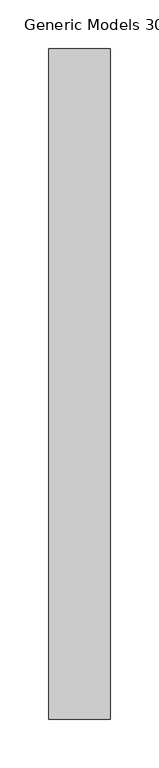
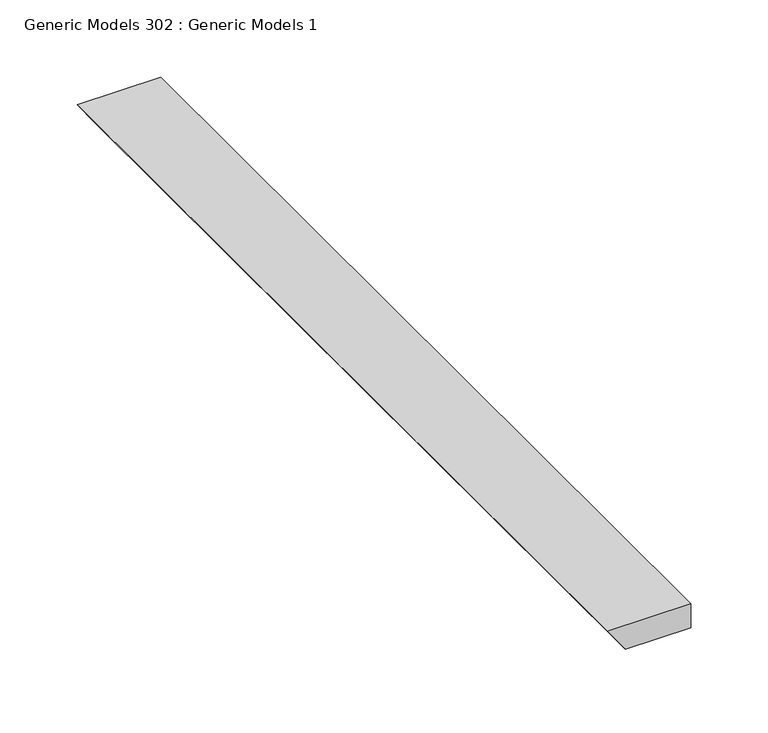
"""IFC4 building model written with IfcOpenShell, lengths in millimetres: proxy geometry, Generic Models 302 : Generic Models 1."""

from ifc_helpers import new_model, si_unit, frame, origin, place, context, project, spatial, polyline, outline, extrude, source, transform, mapped, element, save


def generic_models_302_generic_models_1_691b8c8b(model_context):
    return source(origin(), model_context, "Body", "SweptSolid", [
        extrude(outline(polyline([(124910.8145086, 4830.4400913), (124910.8145086, 4767.9223052), (124891.7645086, 4781.3763704), (124891.7645086, 4830.4400913), (124910.8145086, 4830.4400913)])), frame((0.0, 399.7309662, 0.0), z_axis=(0.0, 1.0, 0.0), x_axis=(0.0, 0.0, 1.0)), (0.0, 0.0, 1.0), 685.546),
    ])


if __name__ == "__main__":
    model = new_model("IFC4")
    model_context = context("Model", 3, world=origin())
    ifc_project = project(units=[si_unit("LENGTHUNIT", "METRE", prefix="MILLI")], contexts=[model_context])
    site = spatial("IfcSite", under=ifc_project)
    building = spatial("IfcBuilding", under=site)
    placement = place(None, origin())
    generic_models_302_generic_models_1_shape = generic_models_302_generic_models_1_691b8c8b(model_context)
    element("IfcBuildingElementProxy", 1, Name="Generic Models 302 : Generic Models 1", ObjectType="Generic Models 302 : Generic Models 1", at=placement, inside=building, context=model_context, shape_type="MappedRepresentation", body=[
        mapped(generic_models_302_generic_models_1_shape, transform((0.0, 0.0, 0.0), x_axis=(1.0, 0.0, 0.0), y_axis=(0.0, 1.0, 0.0), z_axis=(0.0, 0.0, 1.0))),
    ])
    save(model, "model.ifc")

# Revit data of these elements
# Element 1 (IfcBuildingElementProxy, "Generic Models 302 : Generic Models 1")
#   Materials on its faces: "_WOOD FLOORING OR DRYWALL RETURN - DETERMINED BY ARCHITECT"
# Materials
#   "_WOOD FLOORING OR DRYWALL RETURN - DETERMINED BY ARCHITECT": class "Generic", colour RGB 177 130 114, transparency 0, Cost = 0
